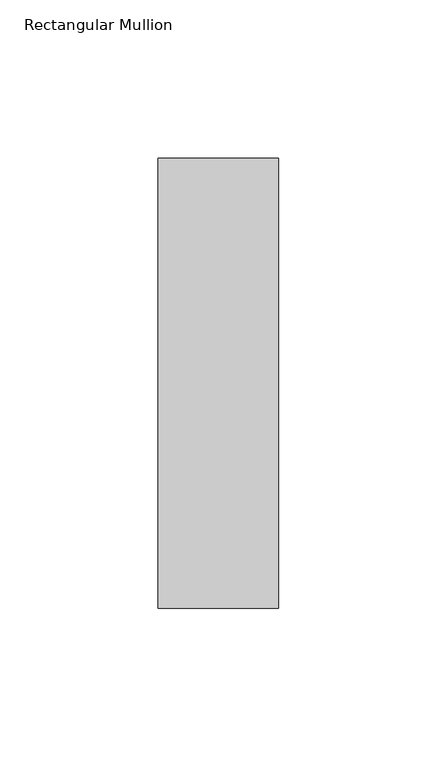
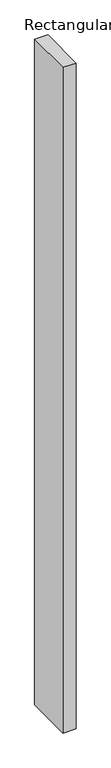
"""IFC4 building model written with IfcOpenShell, lengths in millimetres: member geometry, Rectangular Mullion : NLRS_21_CWM_hsb-regel 38x142_gen_rsf."""

from ifc_helpers import new_model, si_unit, frame, origin, place, context, project, spatial, polyline, outline, extrude, source, transform, mapped, element, save


def rectangular_mullion_df2c1bf7(model_context):
    return source(origin(), model_context, "Body", "SweptSolid", [
        extrude(outline(polyline([(0.0, -71.0), (-38.0, -71.0), (-38.0, 71.0), (0.0, 71.0), (0.0, -71.0)])), frame((0.0, 0.0, -2038.0), z_axis=(0.0, 0.0, 1.0), x_axis=(1.0, 0.0, 0.0)), (0.0, 0.0, 1.0), 2038.0),
    ])


if __name__ == "__main__":
    model = new_model("IFC4")
    model_context = context("Model", 3, world=origin())
    ifc_project = project(units=[si_unit("LENGTHUNIT", "METRE", prefix="MILLI")], contexts=[model_context])
    site = spatial("IfcSite", under=ifc_project)
    building = spatial("IfcBuilding", under=site)
    placement = place(None, origin())
    rectangular_mullion_shape = rectangular_mullion_df2c1bf7(model_context)
    element("IfcMember", 1, ObjectType="Rectangular Mullion : NLRS_21_CWM_hsb-regel 38x142_gen_rsf", at=placement, inside=building, context=model_context, shape_type="MappedRepresentation", body=[
        mapped(rectangular_mullion_shape, transform((0.0, 0.0, 0.0), x_axis=(1.0, 0.0, 0.0), y_axis=(0.0, 1.0, 0.0), z_axis=(0.0, 0.0, 1.0))),
    ])
    save(model, "model.ifc")

# Revit data of these elements
# Type "Rectangular Mullion : NLRS_21_CWM_hsb-regel 38x142_gen_rsf"
#   Export Type to IFC As = "IfcWall"
#   Type IfcGUID = "07M7mRoiH1CR8m_RSKIwpF"
#   Assembly Code = "21.10"
#   built-in parameter 1007322 = 0.465879 (stored number, unit not read)
#   built-in parameter 1007321 = 0.062336 (stored number, unit not read)
#   built-in parameter 1007320 = 0.062336 (stored number, unit not read)
# Element 1 (IfcMember, "Rectangular Mullion : NLRS_21_CWM_hsb-regel 38x142_gen_rsf")
#   Materials on its faces: "NLRS_i2_hout naaldhout vuren_gen_rsf"
# Materials
#   "NLRS_i2_hout naaldhout vuren_gen_rsf": class "I - Hout", colour RGB 234 199 147, transparency 0, Keynote = "i2", Manufacturer = "Revit Standards Foundation", URL = "www.revitstandards.org", Description = "hout vuren", Cost = 0
